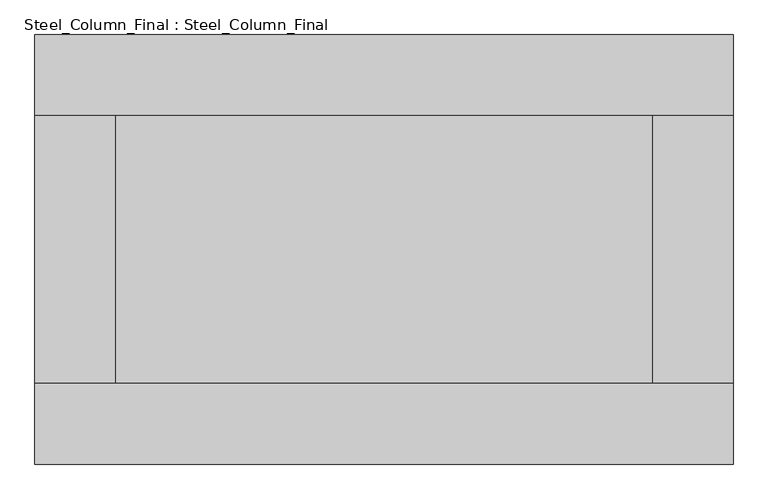
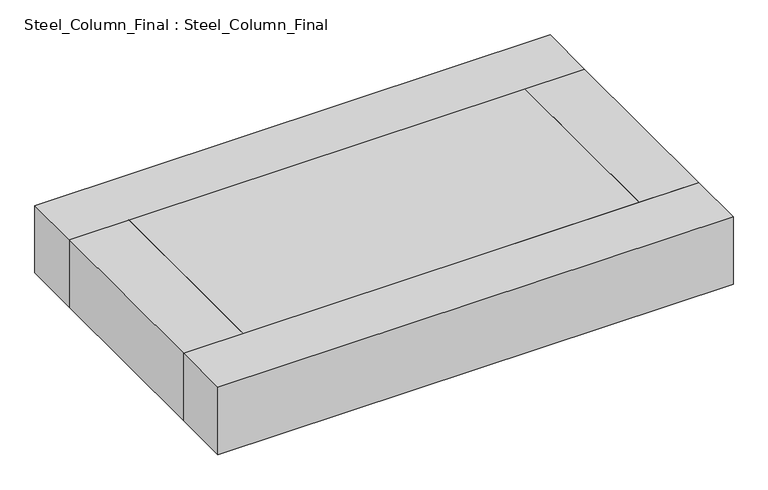
"""IFC4 building model written with IfcOpenShell, lengths in millimetres: proxy geometry, Steel_Column_Final : Steel_Column_Final."""

import ifcopenshell
import ifcopenshell.guid

model = None  # the IFC model being written
_history = None  # IfcOwnerHistory: only IFC2X3 demands one
_inside = {}  # id of a spatial element -> (the spatial element, [elements in it])
_under = {}  # id of a project, library or spatial element -> (it, [spatial elements below it])
_declared = {}  # id of a project -> (the project, [libraries it declares])
_typed = {}  # id of a type object -> (the type object, [elements of that type])
_made_of = {}  # id of a material, layer set ... -> (it, [elements and type objects made of it])


def new_model(schema):
    """Start an empty IFC model of exactly this schema.

    Asked for "IFC4X3", IfcOpenShell would pick the latest addendum, in which some entities
    have other attributes; the version numbers below select the first issue.
    IFC2X3 requires an IfcOwnerHistory on every rooted entity: one is made here for all.
    """
    global model, _history
    if schema == "IFC4X3":
        model = ifcopenshell.file(schema_version=(4, 3, 0, 0))
    else:
        model = ifcopenshell.file(schema=schema)
    _inside.clear()
    _under.clear()
    _declared.clear()
    _typed.clear()
    _made_of.clear()
    _history = None
    if model.schema == "IFC2X3":
        org = make("IfcOrganization", Name="unknown")
        user = make(
            "IfcPersonAndOrganization",
            ThePerson=make("IfcPerson", FamilyName="unknown"),
            TheOrganization=org,
        )
        app = make(
            "IfcApplication",
            ApplicationDeveloper=org,
            Version="unknown",
            ApplicationFullName="unknown",
            ApplicationIdentifier="unknown",
        )
        _history = make(
            "IfcOwnerHistory",
            OwningUser=user,
            OwningApplication=app,
            ChangeAction="ADDED",
            CreationDate=0,
        )
    return model


def make(cls, **values):
    """One entity of the class cls with the attributes given. An attribute that is None is left unset."""
    return model.create_entity(
        cls, **{name: value for name, value in values.items() if value is not None}
    )


def rooted(cls, **values):
    """An entity with a GlobalId (a new one), such as an element, a storey or a relation."""
    return make(cls, GlobalId=ifcopenshell.guid.new(), OwnerHistory=_history, **values)


def si_unit(unit_type, name, prefix=None):
    """IfcSIUnit, for example si_unit("LENGTHUNIT", "METRE", prefix="MILLI")."""
    return make("IfcSIUnit", UnitType=unit_type, Prefix=prefix, Name=name)


def assignment(units):
    """IfcUnitAssignment: the units of a project."""
    return None if units is None else make("IfcUnitAssignment", Units=units)


def point(xyz):
    """IfcCartesianPoint."""
    return None if xyz is None else make("IfcCartesianPoint", Coordinates=xyz)


def direction(xyz):
    """IfcDirection."""
    return None if xyz is None else make("IfcDirection", DirectionRatios=xyz)


def frame(location, z_axis=None, x_axis=None):
    """IfcAxis2Placement3D, a coordinate frame: its origin and axes. An axis left out is left unset."""
    return make(
        "IfcAxis2Placement3D",
        Location=point(location),
        Axis=direction(z_axis),
        RefDirection=direction(x_axis),
    )


def origin():
    """The frame at (0, 0, 0) with its axes left unset."""
    return frame((0.0, 0.0, 0.0))


def place(relative_to, where):
    """IfcLocalPlacement: puts the frame where relative to a parent placement (None: the world)."""
    return make(
        "IfcLocalPlacement", PlacementRelTo=relative_to, RelativePlacement=where
    )


def context(
    kind, dimensions, precision=None, world=None, true_north=None, identifier=None
):
    """IfcGeometricRepresentationContext, for example the 3D "Model" context."""
    return make(
        "IfcGeometricRepresentationContext",
        ContextIdentifier=identifier,
        ContextType=kind,
        CoordinateSpaceDimension=dimensions,
        Precision=precision,
        WorldCoordinateSystem=world,
        TrueNorth=true_north,
    )


def project(units=None, contexts=None):
    """IfcProject with its units and contexts."""
    return rooted(
        "IfcProject",
        Name="project",
        RepresentationContexts=contexts,
        UnitsInContext=assignment(units),
    )


def spatial(cls, under=None, at=None, **own):
    """A site, building, storey or space (cls), placed at a placement, below another one or the project."""
    s = rooted(cls, ObjectPlacement=at, **own)
    if under is not None:
        _under.setdefault(under.id(), (under, []))[1].append(s)
    return s


def polyline(points):
    """IfcPolyline through the points."""
    return make("IfcPolyline", Points=[point(p) for p in points])


def outline(outer, holes=None, kind="AREA"):
    """IfcArbitraryClosedProfileDef: a profile drawn as a closed curve; with holes, ...WithVoids."""
    if holes is None:
        return make("IfcArbitraryClosedProfileDef", ProfileType=kind, OuterCurve=outer)
    return make(
        "IfcArbitraryProfileDefWithVoids",
        ProfileType=kind,
        OuterCurve=outer,
        InnerCurves=holes,
    )


def extrude(swept, where, along, depth):
    """IfcExtrudedAreaSolid: the profile swept, set in the frame where, extruded along a direction by depth."""
    return make(
        "IfcExtrudedAreaSolid",
        SweptArea=swept,
        Position=where,
        ExtrudedDirection=direction(along),
        Depth=depth,
    )


def shape(context_of_items, identifier, shape_type, items):
    """IfcShapeRepresentation: the items that make up one representation, for example the "Body"."""
    return make(
        "IfcShapeRepresentation",
        ContextOfItems=context_of_items,
        RepresentationIdentifier=identifier,
        RepresentationType=shape_type,
        Items=items,
    )


def source(mapping_origin, context_of_items, identifier, shape_type, items):
    """IfcRepresentationMap: a shape defined once, which mapped items show again and again."""
    return make(
        "IfcRepresentationMap",
        MappingOrigin=mapping_origin,
        MappedRepresentation=shape(context_of_items, identifier, shape_type, items),
    )


def transform(
    local_origin,
    x_axis=None,
    y_axis=None,
    z_axis=None,
    scale=None,
    scale2=None,
    scale3=None,
    uniform=True,
):
    """IfcCartesianTransformationOperator3D, or its non-uniform kind. x_axis, y_axis, z_axis: its Axis1, 2, 3."""
    if uniform:
        return make(
            "IfcCartesianTransformationOperator3D",
            Axis1=direction(x_axis),
            Axis2=direction(y_axis),
            LocalOrigin=point(local_origin),
            Scale=scale,
            Axis3=direction(z_axis),
        )
    return make(
        "IfcCartesianTransformationOperator3DnonUniform",
        Axis1=direction(x_axis),
        Axis2=direction(y_axis),
        LocalOrigin=point(local_origin),
        Scale=scale,
        Axis3=direction(z_axis),
        Scale2=scale2,
        Scale3=scale3,
    )


def mapped(mapping_source, mapping_target):
    """IfcMappedItem: shows the shape of a source again, moved by a transform."""
    return make(
        "IfcMappedItem", MappingSource=mapping_source, MappingTarget=mapping_target
    )


def made_of(thing, what):
    """Note that an element or type object is made of a material, layer set ...; save() writes the relation."""
    if what is not None:
        _made_of.setdefault(what.id(), (what, []))[1].append(thing)
    return thing


def element(
    cls,
    number,
    at=None,
    inside=None,
    cuts=None,
    type_object=None,
    material=None,
    context=None,
    identifier="Body",
    shape_type=None,
    held_by="IfcProductDefinitionShape",
    body=None,
    shapes=None,
    **own,
):
    """One element of the class cls, such as IfcWall. Its Tag is "e" and its number.

    at: its placement. inside: the storey or other place that contains it. cuts: it is an
    opening in that element (IfcRelVoidsElement). A single representation is given by context,
    identifier, shape_type and body (its items); several are given by shapes. held_by: the class
    of the entity that holds the representations. save() writes the other relations.
    """
    e = rooted(cls, Tag="e%d" % number, ObjectPlacement=at, **own)
    if body is not None:
        shapes = [shape(context, identifier, shape_type, body)]
    if shapes is not None:
        e.Representation = make(held_by, Representations=shapes)
    if inside is not None:
        _inside.setdefault(inside.id(), (inside, []))[1].append(e)
    if cuts is not None:
        rooted(
            "IfcRelVoidsElement", RelatingBuildingElement=cuts, RelatedOpeningElement=e
        )
    if type_object is not None:
        _typed.setdefault(type_object.id(), (type_object, []))[1].append(e)
    return made_of(e, material)


def aggregate(whole, parts):
    """IfcRelAggregates: a whole, such as a stair, and the parts it consists of."""
    return rooted("IfcRelAggregates", RelatingObject=whole, RelatedObjects=parts)


def save(model, path):
    """Write the relations noted so far, then the file.

    IfcRelAggregates (storeys below a building ...), IfcRelContainedInSpatialStructure (elements
    in a storey), IfcRelDefinesByType, IfcRelAssociatesMaterial and IfcRelDeclares: one each for
    every whole, place, type object, material and project.
    """
    for whole, parts in _under.values():
        aggregate(whole, parts)
    for where, things in _inside.values():
        rooted(
            "IfcRelContainedInSpatialStructure",
            RelatedElements=things,
            RelatingStructure=where,
        )
    for kind, things in _typed.values():
        rooted("IfcRelDefinesByType", RelatedObjects=things, RelatingType=kind)
    for what, things in _made_of.values():
        rooted("IfcRelAssociatesMaterial", RelatedObjects=things, RelatingMaterial=what)
    for by, libraries in _declared.values():
        rooted("IfcRelDeclares", RelatingContext=by, RelatedDefinitions=libraries)
    model.write(path)


def steel_column_final_steel_column_final_5a21aa61(model_context):
    return source(origin(), model_context, "Body", "SweptSolid", [
        extrude(outline(polyline([(6500.0, 2500.0), (-6500.0, 2500.0), (-6500.0, 4000.0), (6500.0, 4000.0), (6500.0, 2500.0)])), frame((0.0, 0.0, 106900.0), z_axis=(0.0, 0.0, 1.0), x_axis=(1.0, 0.0, 0.0)), (0.0, 0.0, 1.0), 1800.0),
        extrude(outline(polyline([(-6500.0, -2500.0), (6500.0, -2500.0), (6500.0, -4000.0), (-6500.0, -4000.0), (-6500.0, -2500.0)])), frame((0.0, 0.0, 106900.0), z_axis=(0.0, 0.0, 1.0), x_axis=(1.0, 0.0, 0.0)), (0.0, 0.0, 1.0), 1800.0),
        extrude(outline(polyline([(5000.0, -2500.0), (5000.0, 2500.0), (6500.0, 2500.0), (6500.0, -2500.0), (5000.0, -2500.0)])), frame((0.0, 0.0, 106900.0), z_axis=(0.0, 0.0, 1.0), x_axis=(1.0, 0.0, 0.0)), (0.0, 0.0, 1.0), 1800.0),
        extrude(outline(polyline([(-5000.0, 2500.0), (-5000.0, -2500.0), (-6500.0, -2500.0), (-6500.0, 2500.0), (-5000.0, 2500.0)])), frame((0.0, 0.0, 106900.0), z_axis=(0.0, 0.0, 1.0), x_axis=(1.0, 0.0, 0.0)), (0.0, 0.0, 1.0), 1800.0),
        extrude(outline(polyline([(-5000.0, -2500.0), (-5000.0, 2500.0), (5000.0, 2500.0), (5000.0, -2500.0), (-5000.0, -2500.0)])), frame((0.0, 0.0, 106900.0), z_axis=(0.0, 0.0, 1.0), x_axis=(1.0, 0.0, 0.0)), (0.0, 0.0, 1.0), 1800.0),
    ])


if __name__ == "__main__":
    model = new_model("IFC4")
    model_context = context("Model", 3, world=origin())
    ifc_project = project(units=[si_unit("LENGTHUNIT", "METRE", prefix="MILLI")], contexts=[model_context])
    site = spatial("IfcSite", under=ifc_project)
    building = spatial("IfcBuilding", under=site)
    placement = place(None, origin())
    steel_column_final_steel_column_final_shape = steel_column_final_steel_column_final_5a21aa61(model_context)
    element("IfcBuildingElementProxy", 1, Name="Steel_Column_Final : Steel_Column_Final", ObjectType="Steel_Column_Final : Steel_Column_Final", at=placement, inside=building, context=model_context, shape_type="MappedRepresentation", body=[
        mapped(steel_column_final_steel_column_final_shape, transform((0.0, 0.0, 0.0), x_axis=(1.0, 0.0, 0.0), y_axis=(0.0, 1.0, 0.0), z_axis=(0.0, 0.0, 1.0))),
    ])
    save(model, "model.ifc")

# Revit data of these elements
# Type "Steel_Column_Final : Steel_Column_Final"
#   Top Width [instance default] = 5000 mm
#   Top Length = 10000 mm
#   Length = 21000 mm
#   Height [instance default] = 50000 mm
#   Bottom Width [instance default] = 5000 mm
#   Default Elevation = 0
# Element 1 (IfcBuildingElementProxy, "Steel_Column_Final : Steel_Column_Final")
#   Height = 106900 mm
